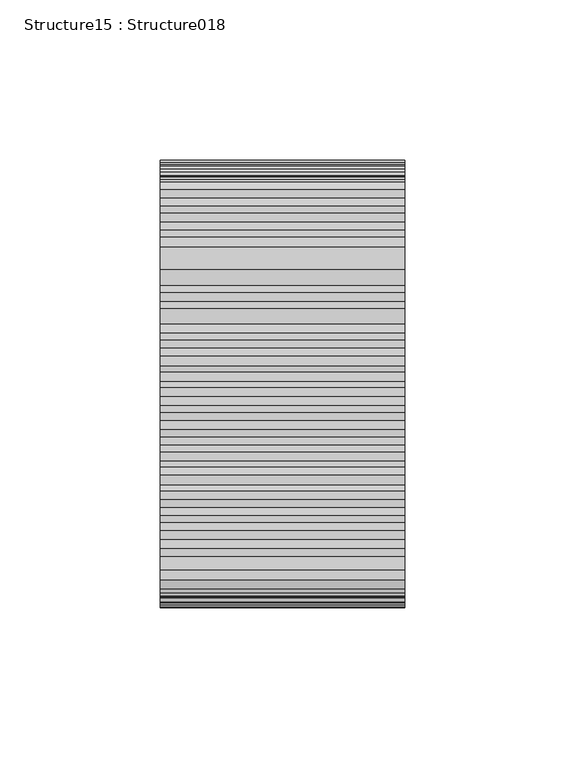
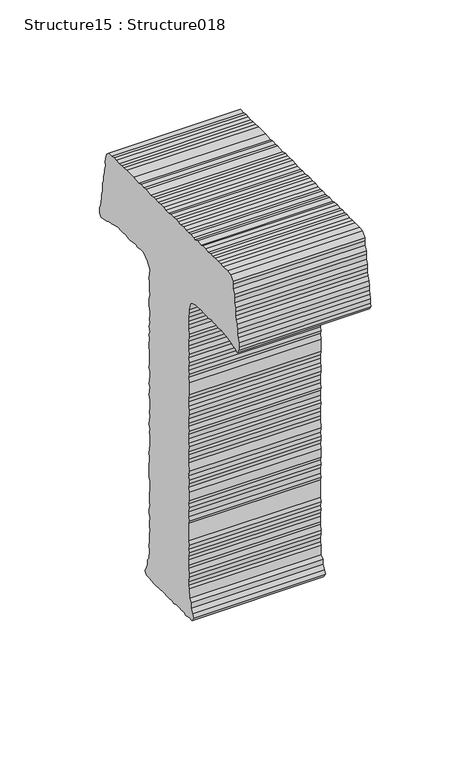
"""IFC4 building model written with IfcOpenShell, lengths in millimetres: proxy geometry, Structure15 : Structure018."""

from ifc_helpers import new_model, si_unit, frame, origin, place, context, project, spatial, polyline, outline, extrude, source, transform, mapped, element, save


def structure15_structure018_85d0241c(model_context):
    return source(origin(), model_context, "Body", "SweptSolid", [
        extrude(outline(polyline([(3.0713309, 0.0), (5.911047, -1.5109738), (7.8963265, -2.6030494), (9.4238315, -4.5682609), (11.8358464, -6.0854453), (13.3694429, -7.1778204), (16.0119655, -8.4761862), (17.5382684, -10.4402037), (20.1734023, -11.3168625), (21.4806426, -12.6154624), (23.4598344, -14.5815725), (26.0843818, -15.8787998), (27.4048447, -17.190535), (30.0308779, -18.9358469), (32.006545, -20.0195676), (33.9822119, -21.1032883), (35.9614038, -23.0693984), (36.177243, -25.4726716), (33.7786193, -27.4520995), (31.6024581, -28.7736316), (29.4188485, -29.6554853), (27.4524467, -31.1853904), (25.707962, -32.0735759), (21.5459857, -34.4901669), (19.8136127, -36.6824447), (18.5063088, -38.4360063), (16.5375586, -39.9802965), (14.5842386, -42.3841725), (13.0581598, -43.9204053), (10.8652254, -45.241993), (8.9086682, -47.2115683), (7.8223113, -48.7535317), (5.4170763, -50.7263919), (3.6760569, -52.4789955), (2.6127037, -57.5259259), (3.9259463, -61.8994311), (5.9000423, -63.4126761), (8.0947718, -65.1618144), (9.6408531, -67.1287615), (12.9302904, -70.3964568), (14.9013555, -72.8022968), (17.0951964, -74.1027493), (20.1664598, -77.1537128), (21.9213862, -79.7759276), (23.2388439, -81.0846774), (25.6504898, -83.0325802), (26.7542686, -84.5768663), (29.1632782, -86.0910654), (30.6934193, -88.4899808), (32.4635341, -89.3695078), (34.4321394, -91.7561863), (36.4014828, -93.281428), (37.9443268, -94.8140744), (39.7013696, -96.9905887), (44.7494208, -102.0052741), (46.9381401, -103.7484418), (48.0337365, -105.7156846), (50.0105242, -107.6794065), (53.9653831, -110.7292372), (54.8458107, -112.4827335), (58.7910531, -115.5230114), (60.1120358, -117.7141506), (63.8360178, -121.4135185), (65.8209323, -122.9375104), (67.7913963, -125.3427534), (69.3261394, -126.4195494), (71.520869, -128.1686877), (72.8322352, -130.3502741), (74.6019809, -131.6605195), (76.132491, -133.6287164), (79.8630843, -137.3346519), (81.6226126, -138.6347473), (84.0258996, -140.5910645), (85.3526049, -142.3400857), (86.8822263, -143.8595969), (88.858782, -145.3920033), (94.3497923, -150.84672), (95.4393784, -152.8079922), (98.9548029, -156.300181), (101.3730601, -158.2546514), (104.6630985, -161.5229438), (106.1906034, -163.4881554), (108.3904546, -164.7945785), (109.9266873, -166.3206573), (111.2416597, -168.5058261), (113.4447481, -170.2465499), (115.1955486, -171.9857782), (116.73267, -173.9605427), (118.9291471, -175.6946989), (122.0010115, -178.7462594), (123.9673497, -180.2685159), (125.9497788, -182.6689267), (129.8926726, -185.7235895), (132.0926012, -186.1500075), (134.5031005, -188.1134895), (136.2533813, -188.9733136), (139.5434058, -190.0694496), (139.7682049, -192.4649055), (138.0182295, -194.2265245), (136.4923788, -196.1928745), (134.5367143, -198.6123337), (133.2261732, -199.9315947), (131.2597675, -201.4603016), (127.7687727, -204.9745241), (126.0370047, -207.1685971), (124.0616431, -208.7063196), (122.1044888, -210.676496), (120.8043935, -212.4360242), (118.8294009, -213.5430283), (117.0883814, -215.2956319), (115.3380371, -217.4879692), (113.6051484, -218.802041), (112.3046839, -220.9922876), (109.6747194, -222.7586216), (108.1482715, -224.7255727), (105.3030648, -224.0880325), (104.4224051, -221.9032208), (103.7630018, -219.0581211), (101.5680402, -216.8776674), (101.3336247, -214.4726586), (97.5937838, -210.3264518), (96.7223716, -208.5819115), (94.7524273, -207.0560727), (92.552945, -205.3189312), (91.0167123, -203.7928524), (89.2683973, -201.1772053), (87.7257853, -200.0758743), (85.7529727, -197.6850163), (84.2077245, -196.1499817), (82.0168887, -194.8525144), (80.711765, -193.1082141), (78.7268504, -191.5842221), (77.4154843, -189.4026357), (69.9416759, -181.9782266), (68.1944003, -181.1213877), (66.6638903, -179.1531908), (64.4599132, -176.9637813), (62.4816099, -175.4463569), (60.9547061, -173.4817423), (59.4097455, -172.3947964), (55.6797532, -168.689458), (54.1496121, -166.2905427), (51.9557712, -164.9900902), (50.4135282, -163.4580408), (48.8830181, -161.4898439), (46.6895462, -159.758673), (43.6141569, -155.824723), (41.8557751, -154.5090484), (39.8831946, -152.549506), (38.790891, -151.0333372), (35.9287047, -149.0689568), (34.8357444, -147.5354177), (33.306492, -145.5851882), (30.8869772, -143.6127504), (29.3522342, -142.5359544), (27.8058653, -140.1209186), (26.0613072, -138.8189763), (24.5218372, -136.8585968), (22.0965998, -135.3282771), (20.1276254, -133.372317), (18.8255068, -131.6310019), (17.2764203, -129.6610695), (15.7401876, -128.1349907), (13.5403364, -126.8285676), (8.2735103, -121.5965534), (6.5251953, -118.9809062), (4.5507303, -117.8983797), (3.2287777, -116.1373617), (1.4773762, -114.3975363), (-0.5069373, -112.8741414), (-1.8225107, -110.6883756), (-4.005533, -109.3986701), (-5.5519019, -106.9836343), (-7.5224473, -105.4571984), (-9.2738488, -103.717373), (-11.4769373, -101.9766492), (-12.7871827, -100.675064), (-14.5427101, -98.0522522), (-16.5186647, -96.5204428), (-17.6145745, -95.0006917), (-19.8093041, -93.2515534), (-21.7870063, -91.7347261), (-23.3226379, -90.2092444), (-27.4724231, -87.8112276), (-29.6694834, -88.2498288), (-32.9486974, -90.2333746), (-35.347926, -92.2110074), (-36.6584671, -93.5302683), (-38.1807117, -95.5002007), (-40.3566408, -97.2530482), (-41.8878412, -99.2319961), (-44.2879545, -100.7621412), (-45.3704772, -102.7378042), (-47.339515, -103.8340056), (-49.0770097, -106.4689986), (-50.8302222, -107.7963169), (-55.1766019, -113.496315), (-56.4836777, -115.679994), (-57.5659086, -118.1049438), (-58.6529221, -119.6295368), (-59.9657206, -122.2553339), (-62.5873958, -121.8243239), (-63.6923209, -120.2956169), (-65.6624973, -118.3384626), (-66.9726655, -116.1568723), (-68.0880402, -114.1866998), (-70.0570146, -112.2307397), (-71.8032945, -110.0481992), (-72.4863917, -107.6452772), (-73.7885104, -105.9039621), (-75.1188218, -104.1513586), (-76.8732285, -102.4085479), (-77.9684599, -100.0093888), (-80.1730381, -97.8193821), (-81.7020585, -96.300468), (-82.5829502, -93.6843408), (-84.562142, -91.7182307), (-85.8795998, -90.4094808), (-85.6781099, -86.6785265), (-83.7128249, -84.2698183), (-80.6612644, -81.1979539), (-79.1384228, -79.2274203), (-76.9541349, -77.4661585), (-75.2157556, -75.2786531), (-73.2559611, -73.7433785), (-71.9402985, -71.9814024), (-69.7653353, -70.6598744), (-68.4576625, -68.4755943), (-66.4921495, -66.4970035), (-64.7566206, -65.6178335), (-63.0011547, -62.9827809), (-60.8255944, -61.6606518), (-59.5240093, -60.3504064), (-57.773665, -58.158069), (-56.0330145, -56.8361839), (-54.2830392, -55.0745649), (-52.9753663, -52.8902848), (-50.8000342, -51.1380383), (-49.2688338, -49.1590904), (-47.7433521, -47.6234587), (-45.5674229, -45.8706112), (-43.6019099, -43.8920204), (-42.0767971, -42.7871071), (-39.9041051, -40.5999588), (-39.019149, -38.8412081), (-36.847054, -36.6546608), (-34.8783038, -35.1103707), (-33.3554622, -33.1398373), (-31.8299805, -31.6042056), (-29.4305238, -30.0566903), (-26.3818315, -26.1198066), (-24.6286189, -24.7924884), (-22.8908367, -22.6055841), (-20.9308142, -21.5004268), (-17.8821219, -17.5635433), (-12.8566895, -12.5046735), (-10.4568638, -10.5264398), (-8.9397409, -8.9992225), (-6.9745968, -7.4513501), (-5.2326113, -5.2674271), (-3.9259045, -3.5144665), (-1.7419855, -2.183923), (0.0, 0.0), (3.0713309, 0.0)])), frame((-35624.0862846, 277151.0596564, 4218.2409142), z_axis=(1.0, 0.0, 1.354250045437766e-12), x_axis=(0.0, 0.7047582970288294, -0.7094474911993307)), (0.0, 0.0, 1.0), 76.2),
    ])


if __name__ == "__main__":
    model = new_model("IFC4")
    model_context = context("Model", 3, world=origin())
    ifc_project = project(units=[si_unit("LENGTHUNIT", "METRE", prefix="MILLI")], contexts=[model_context])
    site = spatial("IfcSite", under=ifc_project)
    building = spatial("IfcBuilding", under=site)
    placement = place(None, origin())
    structure15_structure018_shape = structure15_structure018_85d0241c(model_context)
    element("IfcBuildingElementProxy", 1, Name="Structure15 : Structure018", ObjectType="Structure15 : Structure018", at=placement, inside=building, context=model_context, shape_type="MappedRepresentation", body=[
        mapped(structure15_structure018_shape, transform((0.0, 0.0, 0.0), x_axis=(1.0, 0.0, 0.0), y_axis=(0.0, 1.0, 0.0), z_axis=(0.0, 0.0, 1.0))),
    ])
    save(model, "model.ifc")

# Revit data of these elements
# Type "Structure15 : Structure018"
#   NameOverride = "Structure018"
# Element 1 (IfcBuildingElementProxy, "Structure15 : Structure018")
#   Materials on its faces: "BRUSHED ALUMINUM LETTERING"
# Materials
#   "BRUSHED ALUMINUM LETTERING": class "Unassigned", colour RGB 169 181 186, transparency 0, Cost = 0
